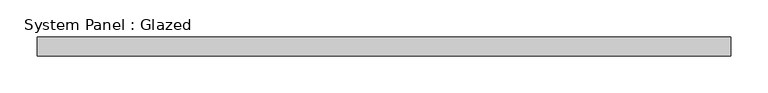
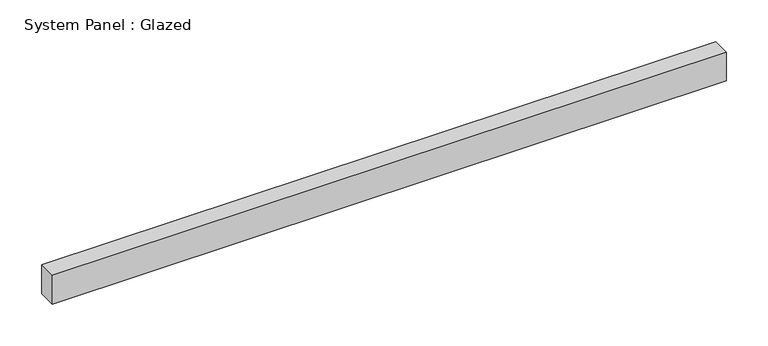
"""IFC4 building model written with IfcOpenShell, lengths in millimetres: plate geometry, System Panel : Glazed."""

import ifcopenshell
import ifcopenshell.guid

model = None  # the IFC model being written
_history = None  # IfcOwnerHistory: only IFC2X3 demands one
_inside = {}  # id of a spatial element -> (the spatial element, [elements in it])
_under = {}  # id of a project, library or spatial element -> (it, [spatial elements below it])
_declared = {}  # id of a project -> (the project, [libraries it declares])
_typed = {}  # id of a type object -> (the type object, [elements of that type])
_made_of = {}  # id of a material, layer set ... -> (it, [elements and type objects made of it])


def new_model(schema):
    """Start an empty IFC model of exactly this schema.

    Asked for "IFC4X3", IfcOpenShell would pick the latest addendum, in which some entities
    have other attributes; the version numbers below select the first issue.
    IFC2X3 requires an IfcOwnerHistory on every rooted entity: one is made here for all.
    """
    global model, _history
    if schema == "IFC4X3":
        model = ifcopenshell.file(schema_version=(4, 3, 0, 0))
    else:
        model = ifcopenshell.file(schema=schema)
    _inside.clear()
    _under.clear()
    _declared.clear()
    _typed.clear()
    _made_of.clear()
    _history = None
    if model.schema == "IFC2X3":
        org = make("IfcOrganization", Name="unknown")
        user = make(
            "IfcPersonAndOrganization",
            ThePerson=make("IfcPerson", FamilyName="unknown"),
            TheOrganization=org,
        )
        app = make(
            "IfcApplication",
            ApplicationDeveloper=org,
            Version="unknown",
            ApplicationFullName="unknown",
            ApplicationIdentifier="unknown",
        )
        _history = make(
            "IfcOwnerHistory",
            OwningUser=user,
            OwningApplication=app,
            ChangeAction="ADDED",
            CreationDate=0,
        )
    return model


def make(cls, **values):
    """One entity of the class cls with the attributes given. An attribute that is None is left unset."""
    return model.create_entity(
        cls, **{name: value for name, value in values.items() if value is not None}
    )


def rooted(cls, **values):
    """An entity with a GlobalId (a new one), such as an element, a storey or a relation."""
    return make(cls, GlobalId=ifcopenshell.guid.new(), OwnerHistory=_history, **values)


def si_unit(unit_type, name, prefix=None):
    """IfcSIUnit, for example si_unit("LENGTHUNIT", "METRE", prefix="MILLI")."""
    return make("IfcSIUnit", UnitType=unit_type, Prefix=prefix, Name=name)


def assignment(units):
    """IfcUnitAssignment: the units of a project."""
    return None if units is None else make("IfcUnitAssignment", Units=units)


def point(xyz):
    """IfcCartesianPoint."""
    return None if xyz is None else make("IfcCartesianPoint", Coordinates=xyz)


def direction(xyz):
    """IfcDirection."""
    return None if xyz is None else make("IfcDirection", DirectionRatios=xyz)


def frame(location, z_axis=None, x_axis=None):
    """IfcAxis2Placement3D, a coordinate frame: its origin and axes. An axis left out is left unset."""
    return make(
        "IfcAxis2Placement3D",
        Location=point(location),
        Axis=direction(z_axis),
        RefDirection=direction(x_axis),
    )


def origin():
    """The frame at (0, 0, 0) with its axes left unset."""
    return frame((0.0, 0.0, 0.0))


def origin_with_axes():
    """The frame at (0, 0, 0) with the z axis (0, 0, 1) and the x axis (1, 0, 0) written out."""
    return frame((0.0, 0.0, 0.0), z_axis=(0.0, 0.0, 1.0), x_axis=(1.0, 0.0, 0.0))


def place(relative_to, where):
    """IfcLocalPlacement: puts the frame where relative to a parent placement (None: the world)."""
    return make(
        "IfcLocalPlacement", PlacementRelTo=relative_to, RelativePlacement=where
    )


def context(
    kind, dimensions, precision=None, world=None, true_north=None, identifier=None
):
    """IfcGeometricRepresentationContext, for example the 3D "Model" context."""
    return make(
        "IfcGeometricRepresentationContext",
        ContextIdentifier=identifier,
        ContextType=kind,
        CoordinateSpaceDimension=dimensions,
        Precision=precision,
        WorldCoordinateSystem=world,
        TrueNorth=true_north,
    )


def project(units=None, contexts=None):
    """IfcProject with its units and contexts."""
    return rooted(
        "IfcProject",
        Name="project",
        RepresentationContexts=contexts,
        UnitsInContext=assignment(units),
    )


def spatial(cls, under=None, at=None, **own):
    """A site, building, storey or space (cls), placed at a placement, below another one or the project."""
    s = rooted(cls, ObjectPlacement=at, **own)
    if under is not None:
        _under.setdefault(under.id(), (under, []))[1].append(s)
    return s


def polyline(points):
    """IfcPolyline through the points."""
    return make("IfcPolyline", Points=[point(p) for p in points])


def outline(outer, holes=None, kind="AREA"):
    """IfcArbitraryClosedProfileDef: a profile drawn as a closed curve; with holes, ...WithVoids."""
    if holes is None:
        return make("IfcArbitraryClosedProfileDef", ProfileType=kind, OuterCurve=outer)
    return make(
        "IfcArbitraryProfileDefWithVoids",
        ProfileType=kind,
        OuterCurve=outer,
        InnerCurves=holes,
    )


def extrude(swept, where, along, depth):
    """IfcExtrudedAreaSolid: the profile swept, set in the frame where, extruded along a direction by depth."""
    return make(
        "IfcExtrudedAreaSolid",
        SweptArea=swept,
        Position=where,
        ExtrudedDirection=direction(along),
        Depth=depth,
    )


def shape(context_of_items, identifier, shape_type, items):
    """IfcShapeRepresentation: the items that make up one representation, for example the "Body"."""
    return make(
        "IfcShapeRepresentation",
        ContextOfItems=context_of_items,
        RepresentationIdentifier=identifier,
        RepresentationType=shape_type,
        Items=items,
    )


def source(mapping_origin, context_of_items, identifier, shape_type, items):
    """IfcRepresentationMap: a shape defined once, which mapped items show again and again."""
    return make(
        "IfcRepresentationMap",
        MappingOrigin=mapping_origin,
        MappedRepresentation=shape(context_of_items, identifier, shape_type, items),
    )


def transform(
    local_origin,
    x_axis=None,
    y_axis=None,
    z_axis=None,
    scale=None,
    scale2=None,
    scale3=None,
    uniform=True,
):
    """IfcCartesianTransformationOperator3D, or its non-uniform kind. x_axis, y_axis, z_axis: its Axis1, 2, 3."""
    if uniform:
        return make(
            "IfcCartesianTransformationOperator3D",
            Axis1=direction(x_axis),
            Axis2=direction(y_axis),
            LocalOrigin=point(local_origin),
            Scale=scale,
            Axis3=direction(z_axis),
        )
    return make(
        "IfcCartesianTransformationOperator3DnonUniform",
        Axis1=direction(x_axis),
        Axis2=direction(y_axis),
        LocalOrigin=point(local_origin),
        Scale=scale,
        Axis3=direction(z_axis),
        Scale2=scale2,
        Scale3=scale3,
    )


def mapped(mapping_source, mapping_target):
    """IfcMappedItem: shows the shape of a source again, moved by a transform."""
    return make(
        "IfcMappedItem", MappingSource=mapping_source, MappingTarget=mapping_target
    )


def made_of(thing, what):
    """Note that an element or type object is made of a material, layer set ...; save() writes the relation."""
    if what is not None:
        _made_of.setdefault(what.id(), (what, []))[1].append(thing)
    return thing


def element(
    cls,
    number,
    at=None,
    inside=None,
    cuts=None,
    type_object=None,
    material=None,
    context=None,
    identifier="Body",
    shape_type=None,
    held_by="IfcProductDefinitionShape",
    body=None,
    shapes=None,
    **own,
):
    """One element of the class cls, such as IfcWall. Its Tag is "e" and its number.

    at: its placement. inside: the storey or other place that contains it. cuts: it is an
    opening in that element (IfcRelVoidsElement). A single representation is given by context,
    identifier, shape_type and body (its items); several are given by shapes. held_by: the class
    of the entity that holds the representations. save() writes the other relations.
    """
    e = rooted(cls, Tag="e%d" % number, ObjectPlacement=at, **own)
    if body is not None:
        shapes = [shape(context, identifier, shape_type, body)]
    if shapes is not None:
        e.Representation = make(held_by, Representations=shapes)
    if inside is not None:
        _inside.setdefault(inside.id(), (inside, []))[1].append(e)
    if cuts is not None:
        rooted(
            "IfcRelVoidsElement", RelatingBuildingElement=cuts, RelatedOpeningElement=e
        )
    if type_object is not None:
        _typed.setdefault(type_object.id(), (type_object, []))[1].append(e)
    return made_of(e, material)


def aggregate(whole, parts):
    """IfcRelAggregates: a whole, such as a stair, and the parts it consists of."""
    return rooted("IfcRelAggregates", RelatingObject=whole, RelatedObjects=parts)


def save(model, path):
    """Write the relations noted so far, then the file.

    IfcRelAggregates (storeys below a building ...), IfcRelContainedInSpatialStructure (elements
    in a storey), IfcRelDefinesByType, IfcRelAssociatesMaterial and IfcRelDeclares: one each for
    every whole, place, type object, material and project.
    """
    for whole, parts in _under.values():
        aggregate(whole, parts)
    for where, things in _inside.values():
        rooted(
            "IfcRelContainedInSpatialStructure",
            RelatedElements=things,
            RelatingStructure=where,
        )
    for kind, things in _typed.values():
        rooted("IfcRelDefinesByType", RelatedObjects=things, RelatingType=kind)
    for what, things in _made_of.values():
        rooted("IfcRelAssociatesMaterial", RelatedObjects=things, RelatingMaterial=what)
    for by, libraries in _declared.values():
        rooted("IfcRelDeclares", RelatingContext=by, RelatedDefinitions=libraries)
    model.write(path)


def system_panel_glazed_c48c36d0(model_context):
    return source(origin(), model_context, "Body", "SweptSolid", [
        extrude(outline(polyline([(465.8483058, -44.45), (-465.8483058, -44.45), (-465.8483058, -19.05), (465.8483058, -19.05), (465.8483058, -44.45)])), origin_with_axes(), (0.0, 0.0, 1.0), 41.9143134),
    ])


if __name__ == "__main__":
    model = new_model("IFC4")
    model_context = context("Model", 3, world=origin())
    ifc_project = project(units=[si_unit("LENGTHUNIT", "METRE", prefix="MILLI")], contexts=[model_context])
    site = spatial("IfcSite", under=ifc_project)
    building = spatial("IfcBuilding", under=site)
    placement = place(None, origin())
    system_panel_glazed_shape = system_panel_glazed_c48c36d0(model_context)
    element("IfcPlate", 1, ObjectType="System Panel : Glazed", at=placement, inside=building, context=model_context, shape_type="MappedRepresentation", body=[
        mapped(system_panel_glazed_shape, transform((0.0, 0.0, 0.0), x_axis=(1.0, 0.0, 0.0), y_axis=(0.0, 1.0, 0.0), z_axis=(0.0, 0.0, 1.0))),
    ])
    save(model, "model.ifc")

# Revit data of these elements
# Type "System Panel : Glazed"
#   Construction Type Id = "GSP4R"
#   Analytic Construction = "1/8 in Pilkington single glazing"
#   Visual Light Transmittance = 0.9
#   Solar Heat Gain Coefficient = 0.86
#   Heat Transfer Coefficient (U) = 1.18115 BTU/(h·ft²·°F)
#   Define Thermal Properties by = 1
# Element 1 (IfcPlate, "System Panel : Glazed")
#   Materials on its faces: "Glass"
# Materials
#   "Glass": class "Glass", colour RGB 0 128 192, transparency 0.75, Description = "Soda Lime Glass", Cost = 0
